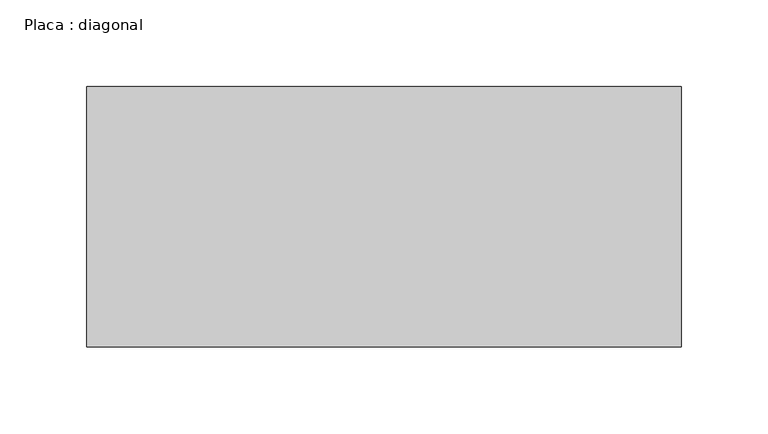
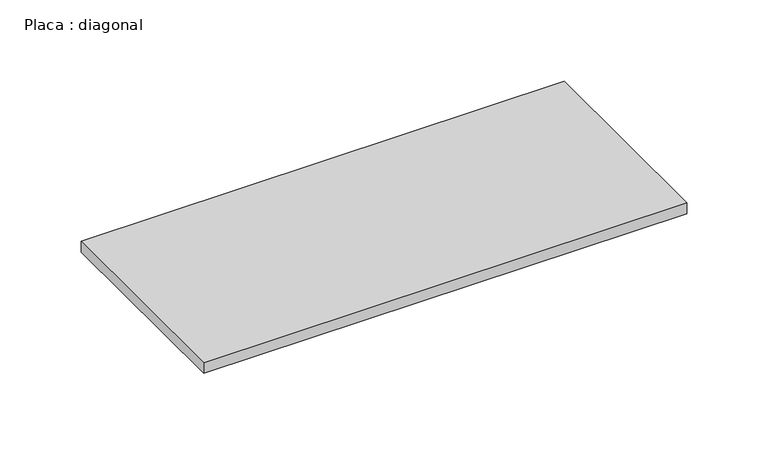
"""IFC4 building model written with IfcOpenShell, lengths in millimetres: beam geometry, Placa : diagonal."""

from ifc_helpers import new_model, si_unit, frame, origin, place, context, project, spatial, polyline, outline, extrude, source, transform, mapped, element, save


def placa_diagonal_b60869c1(model_context):
    return source(origin(), model_context, "Body", "SweptSolid", [
        extrude(outline(polyline([(170.6977773, 75.0), (170.6977773, -75.0), (-171.6122404, -75.0), (-171.6122404, 75.0), (170.6977773, 75.0)])), frame((0.0, 0.0, -4.0), z_axis=(0.0, 0.0, 1.0), x_axis=(1.0, 0.0, 0.0)), (0.0, 0.0, 1.0), 8.0),
    ])


if __name__ == "__main__":
    model = new_model("IFC4")
    model_context = context("Model", 3, world=origin())
    ifc_project = project(units=[si_unit("LENGTHUNIT", "METRE", prefix="MILLI")], contexts=[model_context])
    site = spatial("IfcSite", under=ifc_project)
    building = spatial("IfcBuilding", under=site)
    placement = place(None, origin())
    placa_diagonal_shape = placa_diagonal_b60869c1(model_context)
    element("IfcBeam", 1, ObjectType="Placa : diagonal", at=placement, inside=building, context=model_context, shape_type="MappedRepresentation", body=[
        mapped(placa_diagonal_shape, transform((0.0, 0.0, 0.0), x_axis=(1.0, 0.0, 0.0), y_axis=(0.0, 1.0, 0.0), z_axis=(0.0, 0.0, 1.0))),
    ])
    save(model, "model.ifc")

# Revit data of these elements
# Type "Placa : diagonal"
#   W = 0
#   Length [instance default] = 1.50 m
#   b = 0.15 m
#   d = 0.008 m
#   A = 0 m²
#   Structural Material [instance default] = Aço, 45-345
# Element 1 (IfcBeam, "Placa : diagonal")
#   Materials on its faces: "Aço, 45-345"
# Materials
#   "Aço, 45-345": class "Metal", colour RGB 247 247 247, transparency 0, Description = "Aço 345 MPa", Cost = 0
